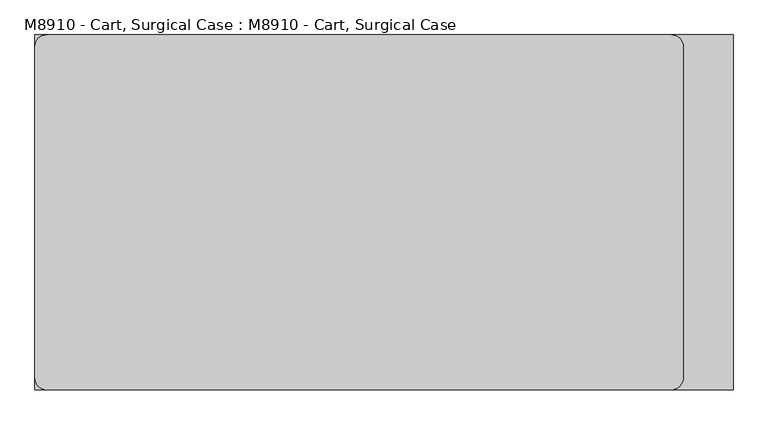
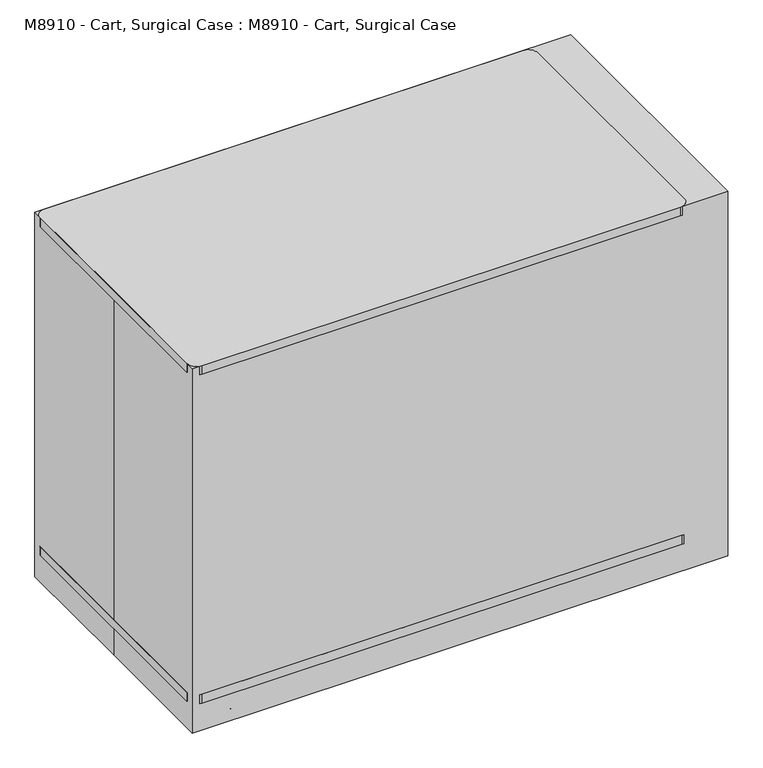
"""IFC4 building model written with IfcOpenShell, lengths in millimetres: proxy geometry, M8910 - Cart, Surgical Case : M8910 - Cart, Surgical Case."""

import ifcopenshell
import ifcopenshell.guid

model = None  # the IFC model being written
_history = None  # IfcOwnerHistory: only IFC2X3 demands one
_inside = {}  # id of a spatial element -> (the spatial element, [elements in it])
_under = {}  # id of a project, library or spatial element -> (it, [spatial elements below it])
_declared = {}  # id of a project -> (the project, [libraries it declares])
_typed = {}  # id of a type object -> (the type object, [elements of that type])
_made_of = {}  # id of a material, layer set ... -> (it, [elements and type objects made of it])


def new_model(schema):
    """Start an empty IFC model of exactly this schema.

    Asked for "IFC4X3", IfcOpenShell would pick the latest addendum, in which some entities
    have other attributes; the version numbers below select the first issue.
    IFC2X3 requires an IfcOwnerHistory on every rooted entity: one is made here for all.
    """
    global model, _history
    if schema == "IFC4X3":
        model = ifcopenshell.file(schema_version=(4, 3, 0, 0))
    else:
        model = ifcopenshell.file(schema=schema)
    _inside.clear()
    _under.clear()
    _declared.clear()
    _typed.clear()
    _made_of.clear()
    _history = None
    if model.schema == "IFC2X3":
        org = make("IfcOrganization", Name="unknown")
        user = make(
            "IfcPersonAndOrganization",
            ThePerson=make("IfcPerson", FamilyName="unknown"),
            TheOrganization=org,
        )
        app = make(
            "IfcApplication",
            ApplicationDeveloper=org,
            Version="unknown",
            ApplicationFullName="unknown",
            ApplicationIdentifier="unknown",
        )
        _history = make(
            "IfcOwnerHistory",
            OwningUser=user,
            OwningApplication=app,
            ChangeAction="ADDED",
            CreationDate=0,
        )
    return model


def make(cls, **values):
    """One entity of the class cls with the attributes given. An attribute that is None is left unset."""
    return model.create_entity(
        cls, **{name: value for name, value in values.items() if value is not None}
    )


def rooted(cls, **values):
    """An entity with a GlobalId (a new one), such as an element, a storey or a relation."""
    return make(cls, GlobalId=ifcopenshell.guid.new(), OwnerHistory=_history, **values)


def si_unit(unit_type, name, prefix=None):
    """IfcSIUnit, for example si_unit("LENGTHUNIT", "METRE", prefix="MILLI")."""
    return make("IfcSIUnit", UnitType=unit_type, Prefix=prefix, Name=name)


def assignment(units):
    """IfcUnitAssignment: the units of a project."""
    return None if units is None else make("IfcUnitAssignment", Units=units)


def point(xyz):
    """IfcCartesianPoint."""
    return None if xyz is None else make("IfcCartesianPoint", Coordinates=xyz)


def direction(xyz):
    """IfcDirection."""
    return None if xyz is None else make("IfcDirection", DirectionRatios=xyz)


def frame(location, z_axis=None, x_axis=None):
    """IfcAxis2Placement3D, a coordinate frame: its origin and axes. An axis left out is left unset."""
    return make(
        "IfcAxis2Placement3D",
        Location=point(location),
        Axis=direction(z_axis),
        RefDirection=direction(x_axis),
    )


def frame_2d(location, x_axis=None):
    """IfcAxis2Placement2D, a coordinate frame in the plane: its origin and x axis."""
    return make(
        "IfcAxis2Placement2D", Location=point(location), RefDirection=direction(x_axis)
    )


def origin():
    """The frame at (0, 0, 0) with its axes left unset."""
    return frame((0.0, 0.0, 0.0))


def origin_with_axes():
    """The frame at (0, 0, 0) with the z axis (0, 0, 1) and the x axis (1, 0, 0) written out."""
    return frame((0.0, 0.0, 0.0), z_axis=(0.0, 0.0, 1.0), x_axis=(1.0, 0.0, 0.0))


def place(relative_to, where):
    """IfcLocalPlacement: puts the frame where relative to a parent placement (None: the world)."""
    return make(
        "IfcLocalPlacement", PlacementRelTo=relative_to, RelativePlacement=where
    )


def context(
    kind, dimensions, precision=None, world=None, true_north=None, identifier=None
):
    """IfcGeometricRepresentationContext, for example the 3D "Model" context."""
    return make(
        "IfcGeometricRepresentationContext",
        ContextIdentifier=identifier,
        ContextType=kind,
        CoordinateSpaceDimension=dimensions,
        Precision=precision,
        WorldCoordinateSystem=world,
        TrueNorth=true_north,
    )


def project(units=None, contexts=None):
    """IfcProject with its units and contexts."""
    return rooted(
        "IfcProject",
        Name="project",
        RepresentationContexts=contexts,
        UnitsInContext=assignment(units),
    )


def spatial(cls, under=None, at=None, **own):
    """A site, building, storey or space (cls), placed at a placement, below another one or the project."""
    s = rooted(cls, ObjectPlacement=at, **own)
    if under is not None:
        _under.setdefault(under.id(), (under, []))[1].append(s)
    return s


def polyline(points):
    """IfcPolyline through the points."""
    return make("IfcPolyline", Points=[point(p) for p in points])


def circle_curve(where, radius):
    """IfcCircle in the frame where."""
    return make("IfcCircle", Position=where, Radius=radius)


def ellipse_curve(where, semi_axis1, semi_axis2):
    """IfcEllipse in the frame where."""
    return make(
        "IfcEllipse", Position=where, SemiAxis1=semi_axis1, SemiAxis2=semi_axis2
    )


def trimmed(basis, trim1, trim2, sense, master):
    """IfcTrimmedCurve: the piece of a basis curve between two trims."""
    return make(
        "IfcTrimmedCurve",
        BasisCurve=basis,
        Trim1=trim1,
        Trim2=trim2,
        SenseAgreement=sense,
        MasterRepresentation=master,
    )


def segment(curve, same_sense, transition):
    """IfcCompositeCurveSegment."""
    return make(
        "IfcCompositeCurveSegment",
        Transition=transition,
        SameSense=same_sense,
        ParentCurve=curve,
    )


def composite_curve(segments, self_intersect=None):
    """IfcCompositeCurve: segments joined end to end."""
    return make("IfcCompositeCurve", Segments=segments, SelfIntersect=self_intersect)


def outline(outer, holes=None, kind="AREA"):
    """IfcArbitraryClosedProfileDef: a profile drawn as a closed curve; with holes, ...WithVoids."""
    if holes is None:
        return make("IfcArbitraryClosedProfileDef", ProfileType=kind, OuterCurve=outer)
    return make(
        "IfcArbitraryProfileDefWithVoids",
        ProfileType=kind,
        OuterCurve=outer,
        InnerCurves=holes,
    )


def extrude(swept, where, along, depth):
    """IfcExtrudedAreaSolid: the profile swept, set in the frame where, extruded along a direction by depth."""
    return make(
        "IfcExtrudedAreaSolid",
        SweptArea=swept,
        Position=where,
        ExtrudedDirection=direction(along),
        Depth=depth,
    )


def shape(context_of_items, identifier, shape_type, items):
    """IfcShapeRepresentation: the items that make up one representation, for example the "Body"."""
    return make(
        "IfcShapeRepresentation",
        ContextOfItems=context_of_items,
        RepresentationIdentifier=identifier,
        RepresentationType=shape_type,
        Items=items,
    )


def source(mapping_origin, context_of_items, identifier, shape_type, items):
    """IfcRepresentationMap: a shape defined once, which mapped items show again and again."""
    return make(
        "IfcRepresentationMap",
        MappingOrigin=mapping_origin,
        MappedRepresentation=shape(context_of_items, identifier, shape_type, items),
    )


def transform(
    local_origin,
    x_axis=None,
    y_axis=None,
    z_axis=None,
    scale=None,
    scale2=None,
    scale3=None,
    uniform=True,
):
    """IfcCartesianTransformationOperator3D, or its non-uniform kind. x_axis, y_axis, z_axis: its Axis1, 2, 3."""
    if uniform:
        return make(
            "IfcCartesianTransformationOperator3D",
            Axis1=direction(x_axis),
            Axis2=direction(y_axis),
            LocalOrigin=point(local_origin),
            Scale=scale,
            Axis3=direction(z_axis),
        )
    return make(
        "IfcCartesianTransformationOperator3DnonUniform",
        Axis1=direction(x_axis),
        Axis2=direction(y_axis),
        LocalOrigin=point(local_origin),
        Scale=scale,
        Axis3=direction(z_axis),
        Scale2=scale2,
        Scale3=scale3,
    )


def mapped(mapping_source, mapping_target):
    """IfcMappedItem: shows the shape of a source again, moved by a transform."""
    return make(
        "IfcMappedItem", MappingSource=mapping_source, MappingTarget=mapping_target
    )


def made_of(thing, what):
    """Note that an element or type object is made of a material, layer set ...; save() writes the relation."""
    if what is not None:
        _made_of.setdefault(what.id(), (what, []))[1].append(thing)
    return thing


def element(
    cls,
    number,
    at=None,
    inside=None,
    cuts=None,
    type_object=None,
    material=None,
    context=None,
    identifier="Body",
    shape_type=None,
    held_by="IfcProductDefinitionShape",
    body=None,
    shapes=None,
    **own,
):
    """One element of the class cls, such as IfcWall. Its Tag is "e" and its number.

    at: its placement. inside: the storey or other place that contains it. cuts: it is an
    opening in that element (IfcRelVoidsElement). A single representation is given by context,
    identifier, shape_type and body (its items); several are given by shapes. held_by: the class
    of the entity that holds the representations. save() writes the other relations.
    """
    e = rooted(cls, Tag="e%d" % number, ObjectPlacement=at, **own)
    if body is not None:
        shapes = [shape(context, identifier, shape_type, body)]
    if shapes is not None:
        e.Representation = make(held_by, Representations=shapes)
    if inside is not None:
        _inside.setdefault(inside.id(), (inside, []))[1].append(e)
    if cuts is not None:
        rooted(
            "IfcRelVoidsElement", RelatingBuildingElement=cuts, RelatedOpeningElement=e
        )
    if type_object is not None:
        _typed.setdefault(type_object.id(), (type_object, []))[1].append(e)
    return made_of(e, material)


def aggregate(whole, parts):
    """IfcRelAggregates: a whole, such as a stair, and the parts it consists of."""
    return rooted("IfcRelAggregates", RelatingObject=whole, RelatedObjects=parts)


def save(model, path):
    """Write the relations noted so far, then the file.

    IfcRelAggregates (storeys below a building ...), IfcRelContainedInSpatialStructure (elements
    in a storey), IfcRelDefinesByType, IfcRelAssociatesMaterial and IfcRelDeclares: one each for
    every whole, place, type object, material and project.
    """
    for whole, parts in _under.values():
        aggregate(whole, parts)
    for where, things in _inside.values():
        rooted(
            "IfcRelContainedInSpatialStructure",
            RelatedElements=things,
            RelatingStructure=where,
        )
    for kind, things in _typed.values():
        rooted("IfcRelDefinesByType", RelatedObjects=things, RelatingType=kind)
    for what, things in _made_of.values():
        rooted("IfcRelAssociatesMaterial", RelatedObjects=things, RelatingMaterial=what)
    for by, libraries in _declared.values():
        rooted("IfcRelDeclares", RelatingContext=by, RelatedDefinitions=libraries)
    model.write(path)


def plane_surface(at):
    """IfcPlane: the flat surface through the origin of the frame at, square to its z axis."""
    return make("IfcPlane", Position=at)


def cylinder_surface(at, radius):
    """IfcCylindricalSurface: all points at the distance radius from the z axis of the frame at."""
    return make("IfcCylindricalSurface", Position=at, Radius=radius)


def advanced_brep(points, edges, surfaces, faces):
    """IfcAdvancedBrep: a solid bounded by faces that lie on surfaces and meet in shared edges.

    An edge is (start, end): straight between two places in points (the first is 0);
    or (start, end, curve); or (start, end, curve, False) where it runs against its curve.
    A face is (place in surfaces, loops), or (place, loops, False) where it looks against
    its surface's normal. A loop lists edges by number (the first is 1), with a minus sign
    where the edge is run from its end to its start. The first loop is the outer one.
    """
    corners = [point(p) for p in points]
    vertices = [make("IfcVertexPoint", VertexGeometry=c) for c in corners]
    made = []
    for start, end, *more in edges:
        made.append(
            make(
                "IfcEdgeCurve",
                EdgeStart=vertices[start],
                EdgeEnd=vertices[end],
                EdgeGeometry=more[0] if more else make("IfcPolyline", Points=[corners[start], corners[end]]),
                SameSense=more[1] if len(more) > 1 else True,
            )
        )
    hull = []
    for where, loops, *sense in faces:
        bounds = []
        for j, loop in enumerate(loops):
            ring = [make("IfcOrientedEdge", EdgeElement=made[abs(k) - 1], Orientation=k > 0) for k in loop]
            bounds.append(
                make(
                    "IfcFaceOuterBound" if j == 0 else "IfcFaceBound",
                    Bound=make("IfcEdgeLoop", EdgeList=ring),
                    Orientation=True,
                )
            )
        hull.append(make("IfcAdvancedFace", Bounds=bounds, FaceSurface=surfaces[where], SameSense=sense[0] if sense else True))
    return make("IfcAdvancedBrep", Outer=make("IfcClosedShell", CfsFaces=hull))


def m8910_cart_surgical_case_m8910_cart_surgical_case_170979ae(model_context):
    return source(origin(), model_context, "Body", "SolidModel", [
        advanced_brep(
        [(596.9, -184.15, 914.4), (596.9, -146.05, 914.4), (704.85, -184.15, 914.4), (666.75, -146.05, 914.4), (704.85, 158.75, 914.4), (666.75, 120.65, 914.4), (596.9, 158.75, 914.4), (596.9, 120.65, 914.4)],
        [
            (0, 1, circle_curve(frame((596.9, -165.1, 914.4), z_axis=(-1.0, 0.0, 0.0), x_axis=(0.0, 1.0, 0.0)), 19.05)),
            (1, 0, circle_curve(frame((596.9, -165.1, 914.4), z_axis=(-1.0, 0.0, 0.0), x_axis=(0.0, 1.0, 0.0)), 19.05)),
            (0, 2),
            (2, 3, ellipse_curve(frame((685.8, -165.1, 914.4), z_axis=(-0.70710678118655, -0.7071067811865451, 0.0), x_axis=(-0.7071067811865449, 0.7071067811865501, 0.0)), 26.9407684, 19.05)),
            (3, 1),
            (3, 2, ellipse_curve(frame((685.8, -165.1, 914.4), z_axis=(-0.70710678118655, -0.7071067811865451, 0.0), x_axis=(-0.7071067811865449, 0.7071067811865501, 0.0)), 26.9407684, 19.05)),
            (2, 4),
            (4, 5, ellipse_curve(frame((685.8, 139.7, 914.4), z_axis=(0.707106781186545, -0.7071067811865499, 0.0), x_axis=(-0.7071067811865498, -0.7071067811865452, 0.0)), 26.9407684, 19.05)),
            (5, 3),
            (5, 4, ellipse_curve(frame((685.8, 139.7, 914.4), z_axis=(0.707106781186545, -0.7071067811865499, 0.0), x_axis=(-0.7071067811865498, -0.7071067811865452, 0.0)), 26.9407684, 19.05)),
            (6, 7, circle_curve(frame((596.9, 139.7, 914.4), z_axis=(-1.0, 0.0, 0.0), x_axis=(0.0, -1.0, 0.0)), 19.05)),
            (7, 6, circle_curve(frame((596.9, 139.7, 914.4), z_axis=(-1.0, 0.0, 0.0), x_axis=(0.0, -1.0, 0.0)), 19.05)),
            (4, 6),
            (7, 5),
        ],
        [
            plane_surface(frame((596.9, -165.1, 0.0), z_axis=(-1.0, 0.0, 0.0), x_axis=(0.0, 0.0, 1.0))),
            cylinder_surface(frame((596.9, -165.1, 914.4), z_axis=(-1.0, 0.0, 0.0), x_axis=(0.0, 1.0, 0.0)), 19.05),
            cylinder_surface(frame((685.8, -165.1, 914.4), z_axis=(0.0, -1.0, 0.0), x_axis=(-1.0, 0.0, 0.0)), 19.05),
            plane_surface(frame((596.9, 139.7, 0.0), z_axis=(-1.0, 0.0, 0.0), x_axis=(0.0, 0.0, 1.0))),
            cylinder_surface(frame((685.8, 139.7, 914.4), z_axis=(1.0, 0.0, 0.0), x_axis=(0.0, -1.0, 0.0)), 19.05),
        ],
        [
            (0, [[1, 2]]),
            (1, [[-1, 3, 4, 5]]),
            (1, [[-2, -5, 6, -3]]),
            (2, [[-4, 7, 8, 9]]),
            (2, [[-6, -9, 10, -7]]),
            (3, [[11, 12]]),
            (4, [[-8, 13, -12, 14]]),
            (4, [[-10, -14, -11, -13]]),
        ],
    ),
        extrude(outline(composite_curve([segment(trimmed(circle_curve(frame_2d((-234.95, 742.95)), 127.0), [point((-336.55, 819.15))], [point((-336.55, 666.75))], True, "CARTESIAN"), True, "CONTINUOUS"), segment(polyline([(-336.55, 666.75), (-336.55, 656.5806623)]), True, "CONTINUOUS"), segment(trimmed(circle_curve(frame_2d((-234.95, 742.95)), 133.35), [point((-336.55, 656.5806623))], [point((-336.55, 829.3193377))], False, "CARTESIAN"), True, "CONTINUOUS"), segment(polyline([(-336.55, 829.3193377), (-336.55, 819.15)]), True, "CONTINUOUS")], self_intersect=False)), frame((-10.0191863, 0.0, 0.0), z_axis=(1.0, 0.0, 0.0), x_axis=(0.0, 1.0, 0.0)), (0.0, 0.0, 1.0), 12.7),
        extrude(outline(polyline([(596.9, -336.55), (-41.7691863, -336.55), (-41.7691863, -323.85), (596.9, -323.85), (596.9, -336.55)])), frame((0.0, 0.0, 107.95), z_axis=(0.0, 0.0, 1.0), x_axis=(1.0, 0.0, 0.0)), (0.0, 0.0, 1.0), 901.7),
        extrude(outline(polyline([(577.85, -323.85), (577.85, 336.55), (596.9, 336.55), (596.9, -323.85), (577.85, -323.85)])), frame((0.0, 0.0, 101.6), z_axis=(0.0, 0.0, 1.0), x_axis=(1.0, 0.0, 0.0)), (0.0, 0.0, 1.0), 914.4),
        extrude(outline(composite_curve([segment(trimmed(circle_curve(frame_2d((595.2202337, 342.9)), 25.4), [point((595.2202337, 368.3))], [point((620.6202337, 342.9))], False, "CARTESIAN"), True, "CONTINUOUS"), segment(polyline([(620.6202337, 342.9), (620.6202337, -343.1423102)]), True, "CONTINUOUS"), segment(trimmed(circle_curve(frame_2d((595.2202337, -343.1423102)), 25.4), [point((620.6202337, -343.1423102))], [point((595.2202337, -368.5423102))], False, "CARTESIAN"), True, "CONTINUOUS"), segment(polyline([(595.2202337, -368.5423102), (-698.5, -368.5423102)]), True, "CONTINUOUS"), segment(trimmed(circle_curve(frame_2d((-698.5, -343.1423102)), 25.4), [point((-698.5, -368.5423102))], [point((-723.9, -343.1423102))], False, "CARTESIAN"), True, "CONTINUOUS"), segment(polyline([(-723.9, -343.1423102), (-723.9, 342.9)]), True, "CONTINUOUS"), segment(trimmed(circle_curve(frame_2d((-698.5, 342.9)), 25.4), [point((-723.9, 342.9))], [point((-698.5, 368.3))], False, "CARTESIAN"), True, "CONTINUOUS"), segment(polyline([(-698.5, 368.3), (595.2202337, 368.3)]), True, "CONTINUOUS")], self_intersect=False)), frame((0.0, 0.0, 1016.0), z_axis=(0.0, 0.0, 1.0), x_axis=(1.0, 0.0, 0.0)), (0.0, 0.0, 1.0), 25.4),
        extrude(outline(polyline([(-679.45, 336.55), (577.85, 336.55), (577.85, 317.5), (-679.45, 317.5), (-679.45, 336.55)])), frame((0.0, 0.0, 101.6), z_axis=(0.0, 0.0, 1.0), x_axis=(1.0, 0.0, 0.0)), (0.0, 0.0, 1.0), 914.4),
        extrude(outline(polyline([(-679.45, 336.55), (-679.45, -323.85), (-698.5, -323.85), (-698.5, 336.55), (-679.45, 336.55)])), frame((0.0, 0.0, 101.6), z_axis=(0.0, 0.0, 1.0), x_axis=(1.0, 0.0, 0.0)), (0.0, 0.0, 1.0), 914.4),
        extrude(outline(polyline([(304.8, 31.75), (292.1, 31.75), (284.2622657, 76.2), (312.6377343, 76.2), (304.8, 31.75)])), frame((-603.25, 0.0, 0.0), z_axis=(1.0, 0.0, 0.0), x_axis=(0.0, 1.0, 0.0)), (0.0, 0.0, 1.0), 3.175),
        extrude(outline(polyline([(304.8, 31.75), (292.1, 31.75), (284.2622657, 76.2), (312.6377343, 76.2), (304.8, 31.75)])), frame((-619.125, 0.0, 0.0), z_axis=(1.0, 0.0, 0.0), x_axis=(0.0, 1.0, 0.0)), (0.0, 0.0, 1.0), 3.175),
        extrude(outline(composite_curve([segment(trimmed(circle_curve(frame_2d((298.45, 31.75)), 31.75), [point((330.2, 31.75))], [point((266.7, 31.75))], False, "CARTESIAN"), True, "CONTINUOUS"), segment(trimmed(circle_curve(frame_2d((298.45, 31.75)), 31.75), [point((266.7, 31.75))], [point((330.2, 31.75))], False, "CARTESIAN"), True, "CONTINUOUS")], self_intersect=False)), frame((-615.95, 0.0, 0.0), z_axis=(1.0, 0.0, 0.0), x_axis=(0.0, 1.0, 0.0)), (0.0, 0.0, 1.0), 12.7),
        extrude(outline(polyline([(304.8, 31.75), (292.1, 31.75), (284.2622657, 76.2), (312.6377343, 76.2), (304.8, 31.75)])), frame((492.125, 0.0, 0.0), z_axis=(1.0, 0.0, 0.0), x_axis=(0.0, 1.0, 0.0)), (0.0, 0.0, 1.0), 3.175),
        extrude(outline(polyline([(304.8, 31.75), (292.1, 31.75), (284.2622657, 76.2), (312.6377343, 76.2), (304.8, 31.75)])), frame((508.0, 0.0, 0.0), z_axis=(1.0, 0.0, 0.0), x_axis=(0.0, 1.0, 0.0)), (0.0, 0.0, 1.0), 3.175),
        extrude(outline(composite_curve([segment(trimmed(circle_curve(frame_2d((298.45, 31.75)), 31.75), [point((330.2, 31.75))], [point((266.7, 31.75))], False, "CARTESIAN"), True, "CONTINUOUS"), segment(trimmed(circle_curve(frame_2d((298.45, 31.75)), 31.75), [point((266.7, 31.75))], [point((330.2, 31.75))], False, "CARTESIAN"), True, "CONTINUOUS")], self_intersect=False)), frame((495.3, 0.0, 0.0), z_axis=(1.0, 0.0, 0.0), x_axis=(0.0, 1.0, 0.0)), (0.0, 0.0, 1.0), 12.7),
        extrude(outline(composite_curve([segment(trimmed(circle_curve(frame_2d((-234.95, 742.95)), 127.0), [point((-336.55, 819.15))], [point((-336.55, 666.75))], True, "CARTESIAN"), True, "CONTINUOUS"), segment(polyline([(-336.55, 666.75), (-336.55, 656.5806623)]), True, "CONTINUOUS"), segment(trimmed(circle_curve(frame_2d((-234.95, 742.95)), 133.35), [point((-336.55, 656.5806623))], [point((-336.55, 829.3193377))], False, "CARTESIAN"), True, "CONTINUOUS"), segment(polyline([(-336.55, 829.3193377), (-336.55, 819.15)]), True, "CONTINUOUS")], self_intersect=False)), frame((-101.6, 0.0, 0.0), z_axis=(1.0, 0.0, 0.0), x_axis=(0.0, 1.0, 0.0)), (0.0, 0.0, 1.0), 12.7),
        extrude(outline(polyline([(-57.15, -336.55), (-698.5, -336.55), (-698.5, -323.85), (-57.15, -323.85), (-57.15, -336.55)])), frame((0.0, 0.0, 107.95), z_axis=(0.0, 0.0, 1.0), x_axis=(1.0, 0.0, 0.0)), (0.0, 0.0, 1.0), 901.7),
        extrude(outline(polyline([(-323.85, 31.75), (-331.6877343, 76.2), (-303.3122657, 76.2), (-311.15, 31.75), (-323.85, 31.75)])), frame((-603.25, 0.0, 0.0), z_axis=(1.0, 0.0, 0.0), x_axis=(0.0, 1.0, 0.0)), (0.0, 0.0, 1.0), 3.175),
        extrude(outline(polyline([(-323.85, 31.75), (-331.6877343, 76.2), (-303.3122657, 76.2), (-311.15, 31.75), (-323.85, 31.75)])), frame((-619.125, 0.0, 0.0), z_axis=(1.0, 0.0, 0.0), x_axis=(0.0, 1.0, 0.0)), (0.0, 0.0, 1.0), 3.175),
        extrude(outline(composite_curve([segment(trimmed(circle_curve(frame_2d((-317.5, 31.75)), 31.75), [point((-349.25, 31.75))], [point((-285.75, 31.75))], False, "CARTESIAN"), True, "CONTINUOUS"), segment(trimmed(circle_curve(frame_2d((-317.5, 31.75)), 31.75), [point((-285.75, 31.75))], [point((-349.25, 31.75))], False, "CARTESIAN"), True, "CONTINUOUS")], self_intersect=False)), frame((-615.95, 0.0, 0.0), z_axis=(1.0, 0.0, 0.0), x_axis=(0.0, 1.0, 0.0)), (0.0, 0.0, 1.0), 12.7),
        extrude(outline(polyline([(-323.85, 31.75), (-331.6877343, 76.2), (-303.3122657, 76.2), (-311.15, 31.75), (-323.85, 31.75)])), frame((492.125, 0.0, 0.0), z_axis=(1.0, 0.0, 0.0), x_axis=(0.0, 1.0, 0.0)), (0.0, 0.0, 1.0), 3.175),
        extrude(outline(polyline([(-323.85, 31.75), (-331.6877343, 76.2), (-303.3122657, 76.2), (-311.15, 31.75), (-323.85, 31.75)])), frame((508.0, 0.0, 0.0), z_axis=(1.0, 0.0, 0.0), x_axis=(0.0, 1.0, 0.0)), (0.0, 0.0, 1.0), 3.175),
        extrude(outline(composite_curve([segment(trimmed(circle_curve(frame_2d((-317.5, 31.75)), 31.75), [point((-349.25, 31.75))], [point((-285.75, 31.75))], False, "CARTESIAN"), True, "CONTINUOUS"), segment(trimmed(circle_curve(frame_2d((-317.5, 31.75)), 31.75), [point((-285.75, 31.75))], [point((-349.25, 31.75))], False, "CARTESIAN"), True, "CONTINUOUS")], self_intersect=False)), frame((495.3, 0.0, 0.0), z_axis=(1.0, 0.0, 0.0), x_axis=(0.0, 1.0, 0.0)), (0.0, 0.0, 1.0), 12.7),
        extrude(outline(composite_curve([segment(trimmed(circle_curve(frame_2d((599.5808137, 342.9)), 25.4), [point((599.5808137, 368.3))], [point((624.9808137, 342.9))], False, "CARTESIAN"), True, "CONTINUOUS"), segment(polyline([(624.9808137, 342.9), (624.9808137, -343.1423102)]), True, "CONTINUOUS"), segment(trimmed(circle_curve(frame_2d((599.5808137, -343.1423102)), 25.4), [point((624.9808137, -343.1423102))], [point((599.5808137, -368.5423102))], False, "CARTESIAN"), True, "CONTINUOUS"), segment(polyline([(599.5808137, -368.5423102), (-698.5, -368.5423102)]), True, "CONTINUOUS"), segment(trimmed(circle_curve(frame_2d((-698.5, -343.1423102)), 25.4), [point((-698.5, -368.5423102))], [point((-723.9, -343.1423102))], False, "CARTESIAN"), True, "CONTINUOUS"), segment(polyline([(-723.9, -343.1423102), (-723.9, 342.9)]), True, "CONTINUOUS"), segment(trimmed(circle_curve(frame_2d((-698.5, 342.9)), 25.4), [point((-723.9, 342.9))], [point((-698.5, 368.3))], False, "CARTESIAN"), True, "CONTINUOUS"), segment(polyline([(-698.5, 368.3), (599.5808137, 368.3)]), True, "CONTINUOUS")], self_intersect=False)), frame((0.0, 0.0, 76.2), z_axis=(0.0, 0.0, 1.0), x_axis=(1.0, 0.0, 0.0)), (0.0, 0.0, 1.0), 25.4),
        extrude(outline(polyline([(-723.9, 368.3), (723.9, 368.3), (723.9, -368.3), (-723.9, -368.3), (-723.9, 0.0), (-723.9, 368.3)])), origin_with_axes(), (0.0, 0.0, 1.0), 1041.4),
    ])


if __name__ == "__main__":
    model = new_model("IFC4")
    model_context = context("Model", 3, world=origin())
    ifc_project = project(units=[si_unit("LENGTHUNIT", "METRE", prefix="MILLI")], contexts=[model_context])
    site = spatial("IfcSite", under=ifc_project)
    building = spatial("IfcBuilding", under=site)
    placement = place(None, origin())
    m8910_cart_surgical_case_m8910_cart_surgical_case_shape = m8910_cart_surgical_case_m8910_cart_surgical_case_170979ae(model_context)
    element("IfcBuildingElementProxy", 1, Name="M8910 - Cart, Surgical Case : M8910 - Cart, Surgical Case", ObjectType="M8910 - Cart, Surgical Case : M8910 - Cart, Surgical Case", at=placement, inside=building, context=model_context, shape_type="MappedRepresentation", body=[
        mapped(m8910_cart_surgical_case_m8910_cart_surgical_case_shape, transform((0.0, 0.0, 0.0), x_axis=(1.0, 0.0, 0.0), y_axis=(0.0, 1.0, 0.0), z_axis=(0.0, 0.0, 1.0))),
    ])
    save(model, "model.ifc")

# Revit data of these elements
# Type "M8910 - Cart, Surgical Case : M8910 - Cart, Surgical Case"
#   Watts2 = "0"
#   Watts1 = "0"
#   Unit_Issue = "EA"
#   UTIL_6_Misc = "-"
#   UTIL_5_NonMedGas = "-"
#   UTIL_4_MiscGas = "-"
#   UTIL_3_MedGas = "-"
#   UTIL_2_Elec = "-"
#   UTIL_1_WaterDrain = "-"
#   Nomenclature = "Cart, Surgical Case"
#   NSN = "6530"
#   Location [instance default] = ""
#   JSN = "M8910"
#   Fund_Source_VA = "-"
#   Fund_Source_Navy = "-"
#   Fund_Source_Army = "-"
#   Fund_Source_AF = "-"
#   ELEC_Volts2 = "0"
#   ELEC_Volts1 = "0"
#   ELEC_Phase2 = "0"
#   ELEC_Phase1 = "0"
#   ELEC_HertzSwitch = "0"
#   ELEC_HertzDependent = "0"
#   ELEC_Hertz = "0"
#   ELEC_Amps2 = "0"
#   ELEC_Amps1 = "0"
#   DetailDescription = "Surgical case cart. Unit consists of two hinged cabinet sections, each section equipped with two pull-out shelves with stops. The entire unit is mounted on four heavy duty conductive swivel casters. Used to transport surgical packs and supplies to surgery and soiled items back to central supply."
#   CAT_VA = "C"
#   CAT_Navy = "C"
#   CAT_IHS = "-"
#   CAT_Army = "C"
#   CAT_AF = "C"
#   BTUperhour = "0"
#   Weight_IP = 285
#   DIM_Width_IP = 4' - 9"
#   DIM_Height_IP = 3' - 5"
#   DIM_Depth_IP = 2' - 5"
#   finish [instance default] = none
# Element 1 (IfcBuildingElementProxy, "M8910 - Cart, Surgical Case : M8910 - Cart, Surgical Case")
#   Materials on its faces: "EquipSpace"
# Materials
#   "EquipSpace": class "Unassigned", colour RGB 221 217 195, transparency 0.5
